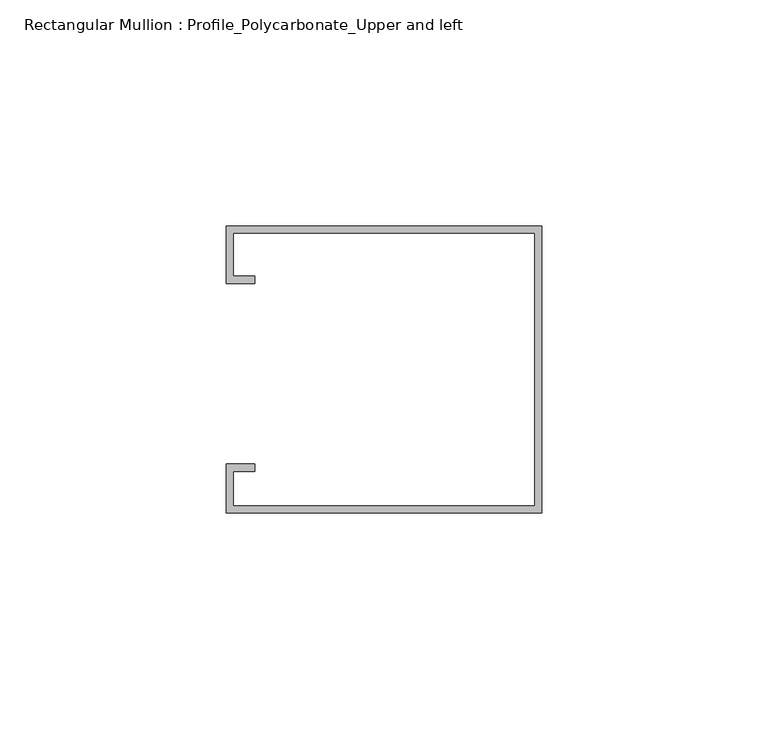
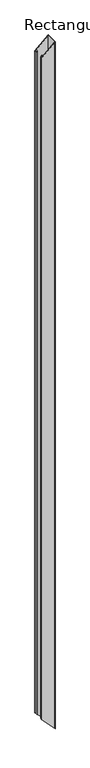
"""IFC4 building model written with IfcOpenShell, lengths in millimetres: member geometry, Rectangular Mullion : Profile_Polycarbonate_Upper and left."""

import ifcopenshell
import ifcopenshell.guid

model = None  # the IFC model being written
_history = None  # IfcOwnerHistory: only IFC2X3 demands one
_inside = {}  # id of a spatial element -> (the spatial element, [elements in it])
_under = {}  # id of a project, library or spatial element -> (it, [spatial elements below it])
_declared = {}  # id of a project -> (the project, [libraries it declares])
_typed = {}  # id of a type object -> (the type object, [elements of that type])
_made_of = {}  # id of a material, layer set ... -> (it, [elements and type objects made of it])


def new_model(schema):
    """Start an empty IFC model of exactly this schema.

    Asked for "IFC4X3", IfcOpenShell would pick the latest addendum, in which some entities
    have other attributes; the version numbers below select the first issue.
    IFC2X3 requires an IfcOwnerHistory on every rooted entity: one is made here for all.
    """
    global model, _history
    if schema == "IFC4X3":
        model = ifcopenshell.file(schema_version=(4, 3, 0, 0))
    else:
        model = ifcopenshell.file(schema=schema)
    _inside.clear()
    _under.clear()
    _declared.clear()
    _typed.clear()
    _made_of.clear()
    _history = None
    if model.schema == "IFC2X3":
        org = make("IfcOrganization", Name="unknown")
        user = make(
            "IfcPersonAndOrganization",
            ThePerson=make("IfcPerson", FamilyName="unknown"),
            TheOrganization=org,
        )
        app = make(
            "IfcApplication",
            ApplicationDeveloper=org,
            Version="unknown",
            ApplicationFullName="unknown",
            ApplicationIdentifier="unknown",
        )
        _history = make(
            "IfcOwnerHistory",
            OwningUser=user,
            OwningApplication=app,
            ChangeAction="ADDED",
            CreationDate=0,
        )
    return model


def make(cls, **values):
    """One entity of the class cls with the attributes given. An attribute that is None is left unset."""
    return model.create_entity(
        cls, **{name: value for name, value in values.items() if value is not None}
    )


def rooted(cls, **values):
    """An entity with a GlobalId (a new one), such as an element, a storey or a relation."""
    return make(cls, GlobalId=ifcopenshell.guid.new(), OwnerHistory=_history, **values)


def si_unit(unit_type, name, prefix=None):
    """IfcSIUnit, for example si_unit("LENGTHUNIT", "METRE", prefix="MILLI")."""
    return make("IfcSIUnit", UnitType=unit_type, Prefix=prefix, Name=name)


def assignment(units):
    """IfcUnitAssignment: the units of a project."""
    return None if units is None else make("IfcUnitAssignment", Units=units)


def point(xyz):
    """IfcCartesianPoint."""
    return None if xyz is None else make("IfcCartesianPoint", Coordinates=xyz)


def direction(xyz):
    """IfcDirection."""
    return None if xyz is None else make("IfcDirection", DirectionRatios=xyz)


def frame(location, z_axis=None, x_axis=None):
    """IfcAxis2Placement3D, a coordinate frame: its origin and axes. An axis left out is left unset."""
    return make(
        "IfcAxis2Placement3D",
        Location=point(location),
        Axis=direction(z_axis),
        RefDirection=direction(x_axis),
    )


def origin():
    """The frame at (0, 0, 0) with its axes left unset."""
    return frame((0.0, 0.0, 0.0))


def place(relative_to, where):
    """IfcLocalPlacement: puts the frame where relative to a parent placement (None: the world)."""
    return make(
        "IfcLocalPlacement", PlacementRelTo=relative_to, RelativePlacement=where
    )


def context(
    kind, dimensions, precision=None, world=None, true_north=None, identifier=None
):
    """IfcGeometricRepresentationContext, for example the 3D "Model" context."""
    return make(
        "IfcGeometricRepresentationContext",
        ContextIdentifier=identifier,
        ContextType=kind,
        CoordinateSpaceDimension=dimensions,
        Precision=precision,
        WorldCoordinateSystem=world,
        TrueNorth=true_north,
    )


def project(units=None, contexts=None):
    """IfcProject with its units and contexts."""
    return rooted(
        "IfcProject",
        Name="project",
        RepresentationContexts=contexts,
        UnitsInContext=assignment(units),
    )


def spatial(cls, under=None, at=None, **own):
    """A site, building, storey or space (cls), placed at a placement, below another one or the project."""
    s = rooted(cls, ObjectPlacement=at, **own)
    if under is not None:
        _under.setdefault(under.id(), (under, []))[1].append(s)
    return s


def faces_of(points, faces, orient=None, outer=None):
    """IfcFace entities. A face is a list of loops; a loop is a list of indices into points, from 0.

    orient and outer hold one flag for each loop. By default every Orientation is true, the
    first loop of a face is its IfcFaceOuterBound and the others are IfcFaceBound.
    """
    made = []
    for i, loops in enumerate(faces):
        bounds = []
        for j, loop in enumerate(loops):
            is_outer = j == 0 if outer is None else outer[i][j]
            bounds.append(
                make(
                    "IfcFaceOuterBound" if is_outer else "IfcFaceBound",
                    Bound=make("IfcPolyLoop", Polygon=[points[k] for k in loop]),
                    Orientation=True if orient is None else orient[i][j],
                )
            )
        made.append(make("IfcFace", Bounds=bounds))
    return made


def faceted_brep(points, faces, orient=None, outer=None, voids=None):
    """IfcFacetedBrep: a solid bounded by flat faces; with voids (closed shells), ...WithVoids."""
    shared = [point(p) for p in points]
    hull = make("IfcClosedShell", CfsFaces=faces_of(shared, faces, orient, outer))
    if voids is None:
        return make("IfcFacetedBrep", Outer=hull)
    return make(
        "IfcFacetedBrepWithVoids",
        Outer=hull,
        Voids=[
            make(cls, CfsFaces=faces_of(shared, fs, o, b)) for cls, fs, o, b in voids
        ],
    )


def shape(context_of_items, identifier, shape_type, items):
    """IfcShapeRepresentation: the items that make up one representation, for example the "Body"."""
    return make(
        "IfcShapeRepresentation",
        ContextOfItems=context_of_items,
        RepresentationIdentifier=identifier,
        RepresentationType=shape_type,
        Items=items,
    )


def source(mapping_origin, context_of_items, identifier, shape_type, items):
    """IfcRepresentationMap: a shape defined once, which mapped items show again and again."""
    return make(
        "IfcRepresentationMap",
        MappingOrigin=mapping_origin,
        MappedRepresentation=shape(context_of_items, identifier, shape_type, items),
    )


def transform(
    local_origin,
    x_axis=None,
    y_axis=None,
    z_axis=None,
    scale=None,
    scale2=None,
    scale3=None,
    uniform=True,
):
    """IfcCartesianTransformationOperator3D, or its non-uniform kind. x_axis, y_axis, z_axis: its Axis1, 2, 3."""
    if uniform:
        return make(
            "IfcCartesianTransformationOperator3D",
            Axis1=direction(x_axis),
            Axis2=direction(y_axis),
            LocalOrigin=point(local_origin),
            Scale=scale,
            Axis3=direction(z_axis),
        )
    return make(
        "IfcCartesianTransformationOperator3DnonUniform",
        Axis1=direction(x_axis),
        Axis2=direction(y_axis),
        LocalOrigin=point(local_origin),
        Scale=scale,
        Axis3=direction(z_axis),
        Scale2=scale2,
        Scale3=scale3,
    )


def mapped(mapping_source, mapping_target):
    """IfcMappedItem: shows the shape of a source again, moved by a transform."""
    return make(
        "IfcMappedItem", MappingSource=mapping_source, MappingTarget=mapping_target
    )


def made_of(thing, what):
    """Note that an element or type object is made of a material, layer set ...; save() writes the relation."""
    if what is not None:
        _made_of.setdefault(what.id(), (what, []))[1].append(thing)
    return thing


def element(
    cls,
    number,
    at=None,
    inside=None,
    cuts=None,
    type_object=None,
    material=None,
    context=None,
    identifier="Body",
    shape_type=None,
    held_by="IfcProductDefinitionShape",
    body=None,
    shapes=None,
    **own,
):
    """One element of the class cls, such as IfcWall. Its Tag is "e" and its number.

    at: its placement. inside: the storey or other place that contains it. cuts: it is an
    opening in that element (IfcRelVoidsElement). A single representation is given by context,
    identifier, shape_type and body (its items); several are given by shapes. held_by: the class
    of the entity that holds the representations. save() writes the other relations.
    """
    e = rooted(cls, Tag="e%d" % number, ObjectPlacement=at, **own)
    if body is not None:
        shapes = [shape(context, identifier, shape_type, body)]
    if shapes is not None:
        e.Representation = make(held_by, Representations=shapes)
    if inside is not None:
        _inside.setdefault(inside.id(), (inside, []))[1].append(e)
    if cuts is not None:
        rooted(
            "IfcRelVoidsElement", RelatingBuildingElement=cuts, RelatedOpeningElement=e
        )
    if type_object is not None:
        _typed.setdefault(type_object.id(), (type_object, []))[1].append(e)
    return made_of(e, material)


def aggregate(whole, parts):
    """IfcRelAggregates: a whole, such as a stair, and the parts it consists of."""
    return rooted("IfcRelAggregates", RelatingObject=whole, RelatedObjects=parts)


def save(model, path):
    """Write the relations noted so far, then the file.

    IfcRelAggregates (storeys below a building ...), IfcRelContainedInSpatialStructure (elements
    in a storey), IfcRelDefinesByType, IfcRelAssociatesMaterial and IfcRelDeclares: one each for
    every whole, place, type object, material and project.
    """
    for whole, parts in _under.values():
        aggregate(whole, parts)
    for where, things in _inside.values():
        rooted(
            "IfcRelContainedInSpatialStructure",
            RelatedElements=things,
            RelatingStructure=where,
        )
    for kind, things in _typed.values():
        rooted("IfcRelDefinesByType", RelatedObjects=things, RelatingType=kind)
    for what, things in _made_of.values():
        rooted("IfcRelAssociatesMaterial", RelatedObjects=things, RelatingMaterial=what)
    for by, libraries in _declared.values():
        rooted("IfcRelDeclares", RelatingContext=by, RelatedDefinitions=libraries)
    model.write(path)


def rectangular_mullion_profile_polycarbonate_upper_and_left_83253e1a(model_context):
    return source(origin(), model_context, "Body", "Brep", [
        faceted_brep([(-69.85, 32.7, -64.2712818), (0.0, 32.7, 0.0), (0.0, 32.7, -3837.5433023), (-69.85, 32.7, -3761.6303539), (-69.85, 20.0, -64.2712818), (-69.85, 20.0, -3761.6303539), (-63.5, 20.0, -58.428438), (-63.5, 20.0, -3768.531531), (-63.5, 21.5875, -58.428438), (-63.5, 21.5875, -3768.531531), (-68.2625, 21.5875, -62.8105708), (-68.2625, 21.5875, -3763.3556482), (-68.2625, 31.1125, -62.8105708), (-68.2625, 31.1125, -3763.3556482), (-1.5875, 31.1125, -1.4607109), (-1.5875, 31.1125, -3835.818008), (-1.5875, -29.2125, -1.4607109), (-1.5875, -29.2125, -3835.818008), (-68.2625, -29.2125, -62.8105708), (-68.2625, -29.2125, -3763.3556482), (-68.2625, -21.5875, -62.8105708), (-68.2625, -21.5875, -3763.3556482), (-63.5, -21.5875, -58.428438), (-63.5, -21.5875, -3768.531531), (-63.5, -20.0, -58.428438), (-63.5, -20.0, -3768.531531), (-69.85, -20.0, -64.2712818), (-69.85, -20.0, -3761.6303539), (-69.85, -30.8, -64.2712818), (-69.85, -30.8, -3761.6303539), (0.0, -30.8, 0.0), (0.0, -30.8, -3837.5433023)], [[[0, 1, 2, 3]], [[4, 0, 3, 5]], [[6, 4, 5, 7]], [[8, 6, 7, 9]], [[10, 8, 9, 11]], [[12, 10, 11, 13]], [[14, 12, 13, 15]], [[16, 14, 15, 17]], [[18, 16, 17, 19]], [[20, 18, 19, 21]], [[22, 20, 21, 23]], [[24, 22, 23, 25]], [[26, 24, 25, 27]], [[28, 26, 27, 29]], [[30, 28, 29, 31]], [[1, 30, 31, 2]], [[1, 0, 4, 6, 8, 10, 12, 14, 16, 18, 20, 22, 24, 26, 28, 30]], [[2, 31, 29, 27, 25, 23, 21, 19, 17, 15, 13, 11, 9, 7, 5, 3]]]),
    ])


if __name__ == "__main__":
    model = new_model("IFC4")
    model_context = context("Model", 3, world=origin())
    ifc_project = project(units=[si_unit("LENGTHUNIT", "METRE", prefix="MILLI")], contexts=[model_context])
    site = spatial("IfcSite", under=ifc_project)
    building = spatial("IfcBuilding", under=site)
    placement = place(None, origin())
    rectangular_mullion_profile_polycarbonate_upper_and_left_shape = rectangular_mullion_profile_polycarbonate_upper_and_left_83253e1a(model_context)
    element("IfcMember", 1, ObjectType="Rectangular Mullion : Profile_Polycarbonate_Upper and left", at=placement, inside=building, context=model_context, shape_type="MappedRepresentation", body=[
        mapped(rectangular_mullion_profile_polycarbonate_upper_and_left_shape, transform((0.0, 0.0, 0.0), x_axis=(1.0, 0.0, 0.0), y_axis=(0.0, 1.0, 0.0), z_axis=(0.0, 0.0, 1.0))),
    ])
    save(model, "model.ifc")

# Revit data of these elements
# Type "Rectangular Mullion : Profile_Polycarbonate_Upper and left"
#   built-in parameter 1007322 = 0.208333 (stored number, unit not read)
#   built-in parameter 1007321 = 0.00520833 (stored number, unit not read)
#   built-in parameter 1007320 = 0 (stored number, unit not read)
# Element 1 (IfcMember, "Rectangular Mullion : Profile_Polycarbonate_Upper and left")
#   Materials on its faces: "ALUMINUM PROFILE AT POLYCARBONATE PANEL"
# Materials
#   "ALUMINUM PROFILE AT POLYCARBONATE PANEL": class "Metal", colour RGB 244 244 244, transparency 0, Description = "Aluminum 6061", Cost = 0
